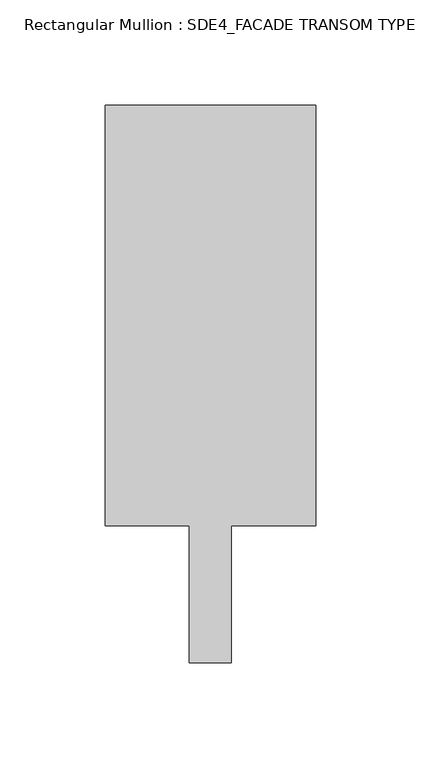
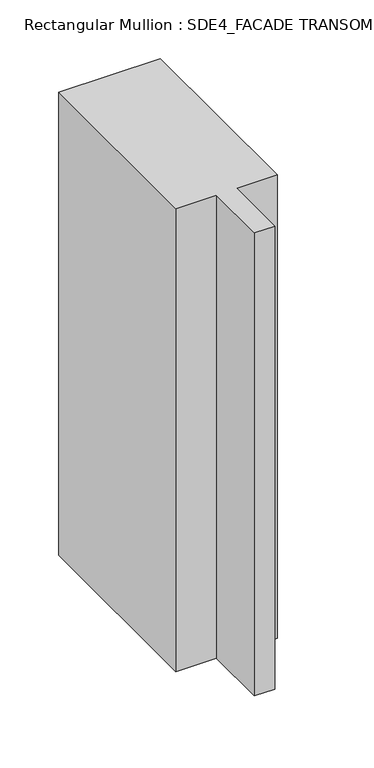
"""IFC4 building model written with IfcOpenShell, lengths in millimetres: member geometry, Rectangular Mullion : SDE4_FACADE TRANSOM TYPE 2."""

import ifcopenshell
import ifcopenshell.guid

model = None  # the IFC model being written
_history = None  # IfcOwnerHistory: only IFC2X3 demands one
_inside = {}  # id of a spatial element -> (the spatial element, [elements in it])
_under = {}  # id of a project, library or spatial element -> (it, [spatial elements below it])
_declared = {}  # id of a project -> (the project, [libraries it declares])
_typed = {}  # id of a type object -> (the type object, [elements of that type])
_made_of = {}  # id of a material, layer set ... -> (it, [elements and type objects made of it])


def new_model(schema):
    """Start an empty IFC model of exactly this schema.

    Asked for "IFC4X3", IfcOpenShell would pick the latest addendum, in which some entities
    have other attributes; the version numbers below select the first issue.
    IFC2X3 requires an IfcOwnerHistory on every rooted entity: one is made here for all.
    """
    global model, _history
    if schema == "IFC4X3":
        model = ifcopenshell.file(schema_version=(4, 3, 0, 0))
    else:
        model = ifcopenshell.file(schema=schema)
    _inside.clear()
    _under.clear()
    _declared.clear()
    _typed.clear()
    _made_of.clear()
    _history = None
    if model.schema == "IFC2X3":
        org = make("IfcOrganization", Name="unknown")
        user = make(
            "IfcPersonAndOrganization",
            ThePerson=make("IfcPerson", FamilyName="unknown"),
            TheOrganization=org,
        )
        app = make(
            "IfcApplication",
            ApplicationDeveloper=org,
            Version="unknown",
            ApplicationFullName="unknown",
            ApplicationIdentifier="unknown",
        )
        _history = make(
            "IfcOwnerHistory",
            OwningUser=user,
            OwningApplication=app,
            ChangeAction="ADDED",
            CreationDate=0,
        )
    return model


def make(cls, **values):
    """One entity of the class cls with the attributes given. An attribute that is None is left unset."""
    return model.create_entity(
        cls, **{name: value for name, value in values.items() if value is not None}
    )


def rooted(cls, **values):
    """An entity with a GlobalId (a new one), such as an element, a storey or a relation."""
    return make(cls, GlobalId=ifcopenshell.guid.new(), OwnerHistory=_history, **values)


def si_unit(unit_type, name, prefix=None):
    """IfcSIUnit, for example si_unit("LENGTHUNIT", "METRE", prefix="MILLI")."""
    return make("IfcSIUnit", UnitType=unit_type, Prefix=prefix, Name=name)


def assignment(units):
    """IfcUnitAssignment: the units of a project."""
    return None if units is None else make("IfcUnitAssignment", Units=units)


def point(xyz):
    """IfcCartesianPoint."""
    return None if xyz is None else make("IfcCartesianPoint", Coordinates=xyz)


def direction(xyz):
    """IfcDirection."""
    return None if xyz is None else make("IfcDirection", DirectionRatios=xyz)


def frame(location, z_axis=None, x_axis=None):
    """IfcAxis2Placement3D, a coordinate frame: its origin and axes. An axis left out is left unset."""
    return make(
        "IfcAxis2Placement3D",
        Location=point(location),
        Axis=direction(z_axis),
        RefDirection=direction(x_axis),
    )


def origin():
    """The frame at (0, 0, 0) with its axes left unset."""
    return frame((0.0, 0.0, 0.0))


def place(relative_to, where):
    """IfcLocalPlacement: puts the frame where relative to a parent placement (None: the world)."""
    return make(
        "IfcLocalPlacement", PlacementRelTo=relative_to, RelativePlacement=where
    )


def context(
    kind, dimensions, precision=None, world=None, true_north=None, identifier=None
):
    """IfcGeometricRepresentationContext, for example the 3D "Model" context."""
    return make(
        "IfcGeometricRepresentationContext",
        ContextIdentifier=identifier,
        ContextType=kind,
        CoordinateSpaceDimension=dimensions,
        Precision=precision,
        WorldCoordinateSystem=world,
        TrueNorth=true_north,
    )


def project(units=None, contexts=None):
    """IfcProject with its units and contexts."""
    return rooted(
        "IfcProject",
        Name="project",
        RepresentationContexts=contexts,
        UnitsInContext=assignment(units),
    )


def spatial(cls, under=None, at=None, **own):
    """A site, building, storey or space (cls), placed at a placement, below another one or the project."""
    s = rooted(cls, ObjectPlacement=at, **own)
    if under is not None:
        _under.setdefault(under.id(), (under, []))[1].append(s)
    return s


def polyline(points):
    """IfcPolyline through the points."""
    return make("IfcPolyline", Points=[point(p) for p in points])


def outline(outer, holes=None, kind="AREA"):
    """IfcArbitraryClosedProfileDef: a profile drawn as a closed curve; with holes, ...WithVoids."""
    if holes is None:
        return make("IfcArbitraryClosedProfileDef", ProfileType=kind, OuterCurve=outer)
    return make(
        "IfcArbitraryProfileDefWithVoids",
        ProfileType=kind,
        OuterCurve=outer,
        InnerCurves=holes,
    )


def extrude(swept, where, along, depth):
    """IfcExtrudedAreaSolid: the profile swept, set in the frame where, extruded along a direction by depth."""
    return make(
        "IfcExtrudedAreaSolid",
        SweptArea=swept,
        Position=where,
        ExtrudedDirection=direction(along),
        Depth=depth,
    )


def shape(context_of_items, identifier, shape_type, items):
    """IfcShapeRepresentation: the items that make up one representation, for example the "Body"."""
    return make(
        "IfcShapeRepresentation",
        ContextOfItems=context_of_items,
        RepresentationIdentifier=identifier,
        RepresentationType=shape_type,
        Items=items,
    )


def source(mapping_origin, context_of_items, identifier, shape_type, items):
    """IfcRepresentationMap: a shape defined once, which mapped items show again and again."""
    return make(
        "IfcRepresentationMap",
        MappingOrigin=mapping_origin,
        MappedRepresentation=shape(context_of_items, identifier, shape_type, items),
    )


def transform(
    local_origin,
    x_axis=None,
    y_axis=None,
    z_axis=None,
    scale=None,
    scale2=None,
    scale3=None,
    uniform=True,
):
    """IfcCartesianTransformationOperator3D, or its non-uniform kind. x_axis, y_axis, z_axis: its Axis1, 2, 3."""
    if uniform:
        return make(
            "IfcCartesianTransformationOperator3D",
            Axis1=direction(x_axis),
            Axis2=direction(y_axis),
            LocalOrigin=point(local_origin),
            Scale=scale,
            Axis3=direction(z_axis),
        )
    return make(
        "IfcCartesianTransformationOperator3DnonUniform",
        Axis1=direction(x_axis),
        Axis2=direction(y_axis),
        LocalOrigin=point(local_origin),
        Scale=scale,
        Axis3=direction(z_axis),
        Scale2=scale2,
        Scale3=scale3,
    )


def mapped(mapping_source, mapping_target):
    """IfcMappedItem: shows the shape of a source again, moved by a transform."""
    return make(
        "IfcMappedItem", MappingSource=mapping_source, MappingTarget=mapping_target
    )


def made_of(thing, what):
    """Note that an element or type object is made of a material, layer set ...; save() writes the relation."""
    if what is not None:
        _made_of.setdefault(what.id(), (what, []))[1].append(thing)
    return thing


def element(
    cls,
    number,
    at=None,
    inside=None,
    cuts=None,
    type_object=None,
    material=None,
    context=None,
    identifier="Body",
    shape_type=None,
    held_by="IfcProductDefinitionShape",
    body=None,
    shapes=None,
    **own,
):
    """One element of the class cls, such as IfcWall. Its Tag is "e" and its number.

    at: its placement. inside: the storey or other place that contains it. cuts: it is an
    opening in that element (IfcRelVoidsElement). A single representation is given by context,
    identifier, shape_type and body (its items); several are given by shapes. held_by: the class
    of the entity that holds the representations. save() writes the other relations.
    """
    e = rooted(cls, Tag="e%d" % number, ObjectPlacement=at, **own)
    if body is not None:
        shapes = [shape(context, identifier, shape_type, body)]
    if shapes is not None:
        e.Representation = make(held_by, Representations=shapes)
    if inside is not None:
        _inside.setdefault(inside.id(), (inside, []))[1].append(e)
    if cuts is not None:
        rooted(
            "IfcRelVoidsElement", RelatingBuildingElement=cuts, RelatedOpeningElement=e
        )
    if type_object is not None:
        _typed.setdefault(type_object.id(), (type_object, []))[1].append(e)
    return made_of(e, material)


def aggregate(whole, parts):
    """IfcRelAggregates: a whole, such as a stair, and the parts it consists of."""
    return rooted("IfcRelAggregates", RelatingObject=whole, RelatedObjects=parts)


def save(model, path):
    """Write the relations noted so far, then the file.

    IfcRelAggregates (storeys below a building ...), IfcRelContainedInSpatialStructure (elements
    in a storey), IfcRelDefinesByType, IfcRelAssociatesMaterial and IfcRelDeclares: one each for
    every whole, place, type object, material and project.
    """
    for whole, parts in _under.values():
        aggregate(whole, parts)
    for where, things in _inside.values():
        rooted(
            "IfcRelContainedInSpatialStructure",
            RelatedElements=things,
            RelatingStructure=where,
        )
    for kind, things in _typed.values():
        rooted("IfcRelDefinesByType", RelatedObjects=things, RelatingType=kind)
    for what, things in _made_of.values():
        rooted("IfcRelAssociatesMaterial", RelatedObjects=things, RelatingMaterial=what)
    for by, libraries in _declared.values():
        rooted("IfcRelDeclares", RelatingContext=by, RelatedDefinitions=libraries)
    model.write(path)


def rectangular_mullion_sde4_facade_transom_type_2_953680b4(model_context):
    return source(origin(), model_context, "Body", "SweptSolid", [
        extrude(outline(polyline([(50.0, 132.5), (50.0, -67.5), (10.0, -67.5), (10.0, -132.5), (-10.0, -132.5), (-10.0, -67.5), (-50.0, -67.5), (-50.0, 132.5), (50.0, 132.5)])), frame((0.0, 0.0, -482.56364), z_axis=(0.0, 0.0, 1.0), x_axis=(1.0, 0.0, 0.0)), (0.0, 0.0, 1.0), 482.56364),
    ])


if __name__ == "__main__":
    model = new_model("IFC4")
    model_context = context("Model", 3, world=origin())
    ifc_project = project(units=[si_unit("LENGTHUNIT", "METRE", prefix="MILLI")], contexts=[model_context])
    site = spatial("IfcSite", under=ifc_project)
    building = spatial("IfcBuilding", under=site)
    placement = place(None, origin())
    rectangular_mullion_sde4_facade_transom_type_2_shape = rectangular_mullion_sde4_facade_transom_type_2_953680b4(model_context)
    element("IfcMember", 1, ObjectType="Rectangular Mullion : SDE4_FACADE TRANSOM TYPE 2", at=placement, inside=building, context=model_context, shape_type="MappedRepresentation", body=[
        mapped(rectangular_mullion_sde4_facade_transom_type_2_shape, transform((0.0, 0.0, 0.0), x_axis=(1.0, 0.0, 0.0), y_axis=(0.0, 1.0, 0.0), z_axis=(0.0, 0.0, 1.0))),
    ])
    save(model, "model.ifc")

# Revit data of these elements
# Type "Rectangular Mullion : SDE4_FACADE TRANSOM TYPE 2"
#   built-in parameter 1007322 = 0.869423 (stored number, unit not read)
#   built-in parameter 1007321 = 0.164042 (stored number, unit not read)
#   built-in parameter 1007320 = 0.164042 (stored number, unit not read)
